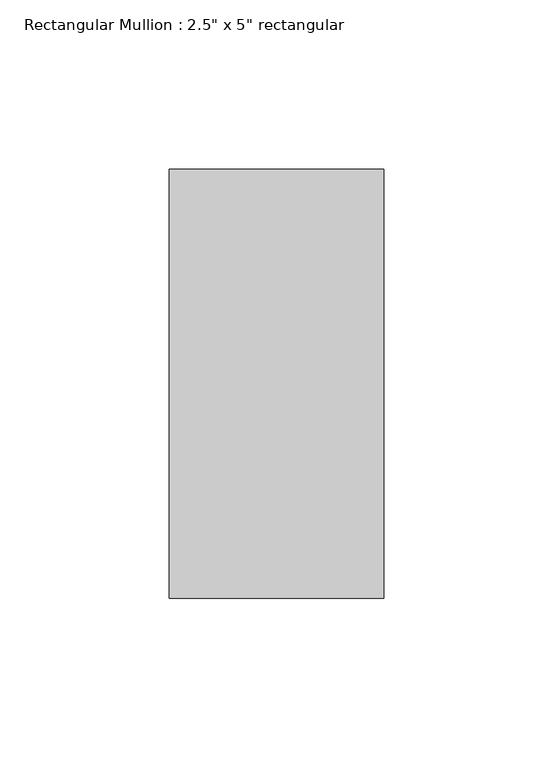
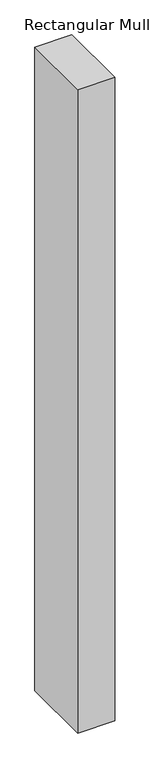
"""IFC4 building model written with IfcOpenShell, lengths in millimetres: member geometry."""

import ifcopenshell
import ifcopenshell.guid

model = None  # the IFC model being written
_history = None  # IfcOwnerHistory: only IFC2X3 demands one
_inside = {}  # id of a spatial element -> (the spatial element, [elements in it])
_under = {}  # id of a project, library or spatial element -> (it, [spatial elements below it])
_declared = {}  # id of a project -> (the project, [libraries it declares])
_typed = {}  # id of a type object -> (the type object, [elements of that type])
_made_of = {}  # id of a material, layer set ... -> (it, [elements and type objects made of it])


def new_model(schema):
    """Start an empty IFC model of exactly this schema.

    Asked for "IFC4X3", IfcOpenShell would pick the latest addendum, in which some entities
    have other attributes; the version numbers below select the first issue.
    IFC2X3 requires an IfcOwnerHistory on every rooted entity: one is made here for all.
    """
    global model, _history
    if schema == "IFC4X3":
        model = ifcopenshell.file(schema_version=(4, 3, 0, 0))
    else:
        model = ifcopenshell.file(schema=schema)
    _inside.clear()
    _under.clear()
    _declared.clear()
    _typed.clear()
    _made_of.clear()
    _history = None
    if model.schema == "IFC2X3":
        org = make("IfcOrganization", Name="unknown")
        user = make(
            "IfcPersonAndOrganization",
            ThePerson=make("IfcPerson", FamilyName="unknown"),
            TheOrganization=org,
        )
        app = make(
            "IfcApplication",
            ApplicationDeveloper=org,
            Version="unknown",
            ApplicationFullName="unknown",
            ApplicationIdentifier="unknown",
        )
        _history = make(
            "IfcOwnerHistory",
            OwningUser=user,
            OwningApplication=app,
            ChangeAction="ADDED",
            CreationDate=0,
        )
    return model


def make(cls, **values):
    """One entity of the class cls with the attributes given. An attribute that is None is left unset."""
    return model.create_entity(
        cls, **{name: value for name, value in values.items() if value is not None}
    )


def rooted(cls, **values):
    """An entity with a GlobalId (a new one), such as an element, a storey or a relation."""
    return make(cls, GlobalId=ifcopenshell.guid.new(), OwnerHistory=_history, **values)


def si_unit(unit_type, name, prefix=None):
    """IfcSIUnit, for example si_unit("LENGTHUNIT", "METRE", prefix="MILLI")."""
    return make("IfcSIUnit", UnitType=unit_type, Prefix=prefix, Name=name)


def assignment(units):
    """IfcUnitAssignment: the units of a project."""
    return None if units is None else make("IfcUnitAssignment", Units=units)


def point(xyz):
    """IfcCartesianPoint."""
    return None if xyz is None else make("IfcCartesianPoint", Coordinates=xyz)


def direction(xyz):
    """IfcDirection."""
    return None if xyz is None else make("IfcDirection", DirectionRatios=xyz)


def frame(location, z_axis=None, x_axis=None):
    """IfcAxis2Placement3D, a coordinate frame: its origin and axes. An axis left out is left unset."""
    return make(
        "IfcAxis2Placement3D",
        Location=point(location),
        Axis=direction(z_axis),
        RefDirection=direction(x_axis),
    )


def origin():
    """The frame at (0, 0, 0) with its axes left unset."""
    return frame((0.0, 0.0, 0.0))


def place(relative_to, where):
    """IfcLocalPlacement: puts the frame where relative to a parent placement (None: the world)."""
    return make(
        "IfcLocalPlacement", PlacementRelTo=relative_to, RelativePlacement=where
    )


def context(
    kind, dimensions, precision=None, world=None, true_north=None, identifier=None
):
    """IfcGeometricRepresentationContext, for example the 3D "Model" context."""
    return make(
        "IfcGeometricRepresentationContext",
        ContextIdentifier=identifier,
        ContextType=kind,
        CoordinateSpaceDimension=dimensions,
        Precision=precision,
        WorldCoordinateSystem=world,
        TrueNorth=true_north,
    )


def project(units=None, contexts=None):
    """IfcProject with its units and contexts."""
    return rooted(
        "IfcProject",
        Name="project",
        RepresentationContexts=contexts,
        UnitsInContext=assignment(units),
    )


def spatial(cls, under=None, at=None, **own):
    """A site, building, storey or space (cls), placed at a placement, below another one or the project."""
    s = rooted(cls, ObjectPlacement=at, **own)
    if under is not None:
        _under.setdefault(under.id(), (under, []))[1].append(s)
    return s


def polyline(points):
    """IfcPolyline through the points."""
    return make("IfcPolyline", Points=[point(p) for p in points])


def outline(outer, holes=None, kind="AREA"):
    """IfcArbitraryClosedProfileDef: a profile drawn as a closed curve; with holes, ...WithVoids."""
    if holes is None:
        return make("IfcArbitraryClosedProfileDef", ProfileType=kind, OuterCurve=outer)
    return make(
        "IfcArbitraryProfileDefWithVoids",
        ProfileType=kind,
        OuterCurve=outer,
        InnerCurves=holes,
    )


def extrude(swept, where, along, depth):
    """IfcExtrudedAreaSolid: the profile swept, set in the frame where, extruded along a direction by depth."""
    return make(
        "IfcExtrudedAreaSolid",
        SweptArea=swept,
        Position=where,
        ExtrudedDirection=direction(along),
        Depth=depth,
    )


def shape(context_of_items, identifier, shape_type, items):
    """IfcShapeRepresentation: the items that make up one representation, for example the "Body"."""
    return make(
        "IfcShapeRepresentation",
        ContextOfItems=context_of_items,
        RepresentationIdentifier=identifier,
        RepresentationType=shape_type,
        Items=items,
    )


def source(mapping_origin, context_of_items, identifier, shape_type, items):
    """IfcRepresentationMap: a shape defined once, which mapped items show again and again."""
    return make(
        "IfcRepresentationMap",
        MappingOrigin=mapping_origin,
        MappedRepresentation=shape(context_of_items, identifier, shape_type, items),
    )


def transform(
    local_origin,
    x_axis=None,
    y_axis=None,
    z_axis=None,
    scale=None,
    scale2=None,
    scale3=None,
    uniform=True,
):
    """IfcCartesianTransformationOperator3D, or its non-uniform kind. x_axis, y_axis, z_axis: its Axis1, 2, 3."""
    if uniform:
        return make(
            "IfcCartesianTransformationOperator3D",
            Axis1=direction(x_axis),
            Axis2=direction(y_axis),
            LocalOrigin=point(local_origin),
            Scale=scale,
            Axis3=direction(z_axis),
        )
    return make(
        "IfcCartesianTransformationOperator3DnonUniform",
        Axis1=direction(x_axis),
        Axis2=direction(y_axis),
        LocalOrigin=point(local_origin),
        Scale=scale,
        Axis3=direction(z_axis),
        Scale2=scale2,
        Scale3=scale3,
    )


def mapped(mapping_source, mapping_target):
    """IfcMappedItem: shows the shape of a source again, moved by a transform."""
    return make(
        "IfcMappedItem", MappingSource=mapping_source, MappingTarget=mapping_target
    )


def made_of(thing, what):
    """Note that an element or type object is made of a material, layer set ...; save() writes the relation."""
    if what is not None:
        _made_of.setdefault(what.id(), (what, []))[1].append(thing)
    return thing


def element(
    cls,
    number,
    at=None,
    inside=None,
    cuts=None,
    type_object=None,
    material=None,
    context=None,
    identifier="Body",
    shape_type=None,
    held_by="IfcProductDefinitionShape",
    body=None,
    shapes=None,
    **own,
):
    """One element of the class cls, such as IfcWall. Its Tag is "e" and its number.

    at: its placement. inside: the storey or other place that contains it. cuts: it is an
    opening in that element (IfcRelVoidsElement). A single representation is given by context,
    identifier, shape_type and body (its items); several are given by shapes. held_by: the class
    of the entity that holds the representations. save() writes the other relations.
    """
    e = rooted(cls, Tag="e%d" % number, ObjectPlacement=at, **own)
    if body is not None:
        shapes = [shape(context, identifier, shape_type, body)]
    if shapes is not None:
        e.Representation = make(held_by, Representations=shapes)
    if inside is not None:
        _inside.setdefault(inside.id(), (inside, []))[1].append(e)
    if cuts is not None:
        rooted(
            "IfcRelVoidsElement", RelatingBuildingElement=cuts, RelatedOpeningElement=e
        )
    if type_object is not None:
        _typed.setdefault(type_object.id(), (type_object, []))[1].append(e)
    return made_of(e, material)


def aggregate(whole, parts):
    """IfcRelAggregates: a whole, such as a stair, and the parts it consists of."""
    return rooted("IfcRelAggregates", RelatingObject=whole, RelatedObjects=parts)


def save(model, path):
    """Write the relations noted so far, then the file.

    IfcRelAggregates (storeys below a building ...), IfcRelContainedInSpatialStructure (elements
    in a storey), IfcRelDefinesByType, IfcRelAssociatesMaterial and IfcRelDeclares: one each for
    every whole, place, type object, material and project.
    """
    for whole, parts in _under.values():
        aggregate(whole, parts)
    for where, things in _inside.values():
        rooted(
            "IfcRelContainedInSpatialStructure",
            RelatedElements=things,
            RelatingStructure=where,
        )
    for kind, things in _typed.values():
        rooted("IfcRelDefinesByType", RelatedObjects=things, RelatingType=kind)
    for what, things in _made_of.values():
        rooted("IfcRelAssociatesMaterial", RelatedObjects=things, RelatingMaterial=what)
    for by, libraries in _declared.values():
        rooted("IfcRelDeclares", RelatingContext=by, RelatedDefinitions=libraries)
    model.write(path)


def member_f0de6b6c(model_context):
    return source(origin(), model_context, "Body", "SweptSolid", [
        extrude(outline(polyline([(0.0, 63.5), (0.0, -63.5), (-63.5, -63.5), (-63.5, 63.5), (0.0, 63.5)])), frame((0.0, 0.0, -1166.2833333), z_axis=(0.0, 0.0, 1.0), x_axis=(1.0, 0.0, 0.0)), (0.0, 0.0, 1.0), 1166.2833333),
    ])


if __name__ == "__main__":
    model = new_model("IFC4")
    model_context = context("Model", 3, world=origin())
    ifc_project = project(units=[si_unit("LENGTHUNIT", "METRE", prefix="MILLI")], contexts=[model_context])
    site = spatial("IfcSite", under=ifc_project)
    building = spatial("IfcBuilding", under=site)
    placement = place(None, origin())
    member_shape = member_f0de6b6c(model_context)
    element("IfcMember", 1, ObjectType="Rectangular Mullion : 2.5\" x 5\" rectangular", at=placement, inside=building, context=model_context, shape_type="MappedRepresentation", body=[
        mapped(member_shape, transform((0.0, 0.0, 0.0), x_axis=(1.0, 0.0, 0.0), y_axis=(0.0, 1.0, 0.0), z_axis=(0.0, 0.0, 1.0))),
    ])
    save(model, "model.ifc")

# Revit data of these elements
# Type "Rectangular Mullion : 2.5\" x 5\" rectangular"
#   built-in parameter 1007304 = 0.416667 (stored number, unit not read)
#   built-in parameter 1007301 = 0.104167 (stored number, unit not read)
#   built-in parameter 1007300 = 0.104167 (stored number, unit not read)
